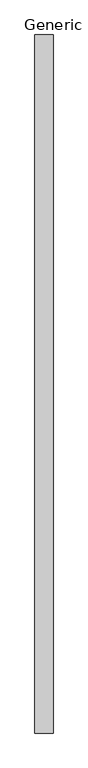
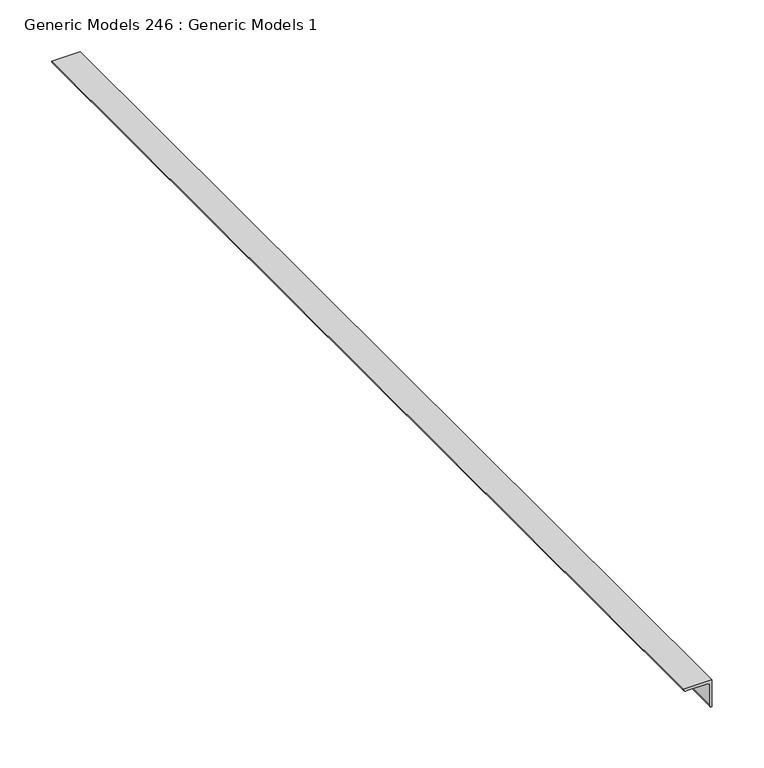
"""IFC4 building model written with IfcOpenShell, lengths in millimetres: proxy geometry, Generic Models 246 : Generic Models 1."""

from ifc_helpers import new_model, si_unit, point, frame, frame_2d, origin, place, context, project, spatial, polyline, circle_curve, trimmed, segment, composite_curve, outline, extrude, source, transform, mapped, element, save


def generic_models_246_generic_models_1_150aa8f0(model_context):
    return source(origin(), model_context, "Body", "SweptSolid", [
        extrude(outline(composite_curve([segment(polyline([(2342.7526794, 50229.5071108), (2342.7526794, 50197.7571108)]), True, "CONTINUOUS"), segment(trimmed(circle_curve(frame_2d((2342.7526794, 50200.9321108)), 3.175), [point((2342.7526794, 50197.7571108))], [point((2339.5776794, 50200.9321108))], False, "CARTESIAN"), True, "CONTINUOUS"), segment(polyline([(2339.5776794, 50200.9321108), (2339.5776794, 50224.7446108)]), True, "CONTINUOUS"), segment(trimmed(circle_curve(frame_2d((2337.9901794, 50224.7446108)), 1.5875), [point((2339.5776794, 50224.7446108))], [point((2337.9901794, 50226.3321108))], True, "CARTESIAN"), True, "CONTINUOUS"), segment(polyline([(2337.9901794, 50226.3321108), (2314.1776794, 50226.3321108)]), True, "CONTINUOUS"), segment(trimmed(circle_curve(frame_2d((2314.1776794, 50229.5071108)), 3.175), [point((2314.1776794, 50226.3321108))], [point((2311.0026794, 50229.5071108))], False, "CARTESIAN"), True, "CONTINUOUS"), segment(polyline([(2311.0026794, 50229.5071108), (2342.7526794, 50229.5071108)]), True, "CONTINUOUS")], self_intersect=False)), frame((0.0, 0.0, 0.0), z_axis=(0.0, 1.0, 0.0), x_axis=(0.0, 0.0, 1.0)), (0.0, 0.0, 1.0), 1219.2),
    ])


if __name__ == "__main__":
    model = new_model("IFC4")
    model_context = context("Model", 3, world=origin())
    ifc_project = project(units=[si_unit("LENGTHUNIT", "METRE", prefix="MILLI")], contexts=[model_context])
    site = spatial("IfcSite", under=ifc_project)
    building = spatial("IfcBuilding", under=site)
    placement = place(None, origin())
    generic_models_246_generic_models_1_shape = generic_models_246_generic_models_1_150aa8f0(model_context)
    element("IfcBuildingElementProxy", 1, Name="Generic Models 246 : Generic Models 1", ObjectType="Generic Models 246 : Generic Models 1", at=placement, inside=building, context=model_context, shape_type="MappedRepresentation", body=[
        mapped(generic_models_246_generic_models_1_shape, transform((0.0, 0.0, 0.0), x_axis=(1.0, 0.0, 0.0), y_axis=(0.0, 1.0, 0.0), z_axis=(0.0, 0.0, 1.0))),
    ])
    save(model, "model.ifc")

# Revit data of these elements
# Element 1 (IfcBuildingElementProxy, "Generic Models 246 : Generic Models 1")
#   Materials on its faces: "BULKHEAD FRAME WORK"
# Materials
#   "BULKHEAD FRAME WORK": class "Metal", colour RGB 189 187 185, transparency 0, Description = "Structural steel 50ksi", Cost = 0
